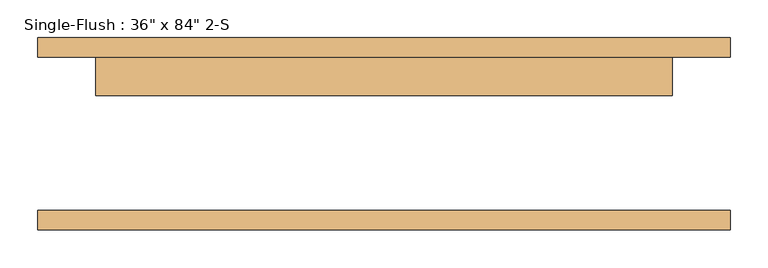
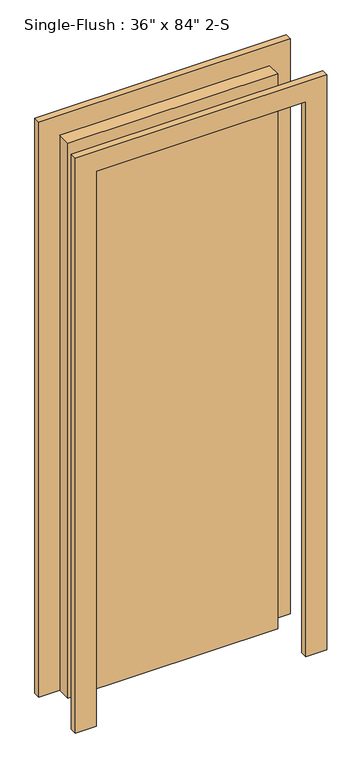
"""IFC4 building model written with IfcOpenShell, lengths in millimetres: door geometry."""

from ifc_helpers import new_model, si_unit, frame, origin, origin_with_axes, place, context, project, spatial, polyline, outline, extrude, source, transform, mapped, element, save


def door_b6acaa4e(model_context):
    return source(origin(), model_context, "Body", "SweptSolid", [
        extrude(outline(polyline([(2209.8, -457.2), (0.0, -457.2), (0.0, -381.0), (2133.6, -381.0), (2133.6, 381.0), (0.0, 381.0), (0.0, 457.2), (2209.8, 457.2), (2209.8, -457.2)])), frame((0.0, 101.6, 0.0), z_axis=(0.0, 1.0, 0.0), x_axis=(0.0, 0.0, 1.0)), (0.0, 0.0, 1.0), 25.4),
        extrude(outline(polyline([(2209.8, 457.2), (2209.8, -457.2), (0.0, -457.2), (0.0, -381.0), (2133.6, -381.0), (2133.6, 381.0), (0.0, 381.0), (0.0, 457.2), (2209.8, 457.2)])), frame((0.0, -127.0, 0.0), z_axis=(0.0, 1.0, 0.0), x_axis=(0.0, 0.0, 1.0)), (0.0, 0.0, 1.0), 25.4),
        extrude(outline(polyline([(381.0, 50.8), (-381.0, 50.8), (-381.0, 101.6), (381.0, 101.6), (381.0, 50.8)])), origin_with_axes(), (0.0, 0.0, 1.0), 2133.6),
    ])


if __name__ == "__main__":
    model = new_model("IFC4")
    model_context = context("Model", 3, world=origin())
    ifc_project = project(units=[si_unit("LENGTHUNIT", "METRE", prefix="MILLI")], contexts=[model_context])
    site = spatial("IfcSite", under=ifc_project)
    building = spatial("IfcBuilding", under=site)
    placement = place(None, origin())
    door_shape = door_b6acaa4e(model_context)
    element("IfcDoor", 1, ObjectType="Single-Flush : 36\" x 84\" 2-S", at=placement, inside=building, context=model_context, shape_type="MappedRepresentation", body=[
        mapped(door_shape, transform((0.0, 0.0, 0.0), x_axis=(1.0, 0.0, 0.0), y_axis=(0.0, 1.0, 0.0), z_axis=(0.0, 0.0, 1.0))),
    ])
    save(model, "model.ifc")

# Revit data of these elements
# Type "Single-Flush : 36\" x 84\" 2-S"
#   Type Mark = "57"
#   Assembly Code = "C1020"
#   Thickness = 0' - 2"
#   Height = 7' - 0"
#   Trim Projection Ext = 0' - 1"
#   Trim Projection Int = 0' - 1"
#   Trim Width = 0' - 3"
#   Width = 2' - 6"
#   Door Material = Door - Panel
#   Frame Material = Door - Frame
#   Wall Closure = (empty or 0)
# Element 1 (IfcDoor, "Single-Flush : 36\" x 84\" 2-S")
#   Materials on its faces: "Door - Frame", "Door - Panel"
# Materials
#   "Door - Panel": class "Wood", colour RGB 227 170 128, transparency 0, Cost = 0
#   "Door - Frame": class "Miscellaneous", colour RGB 153 76 43, transparency 0, Cost = 0
